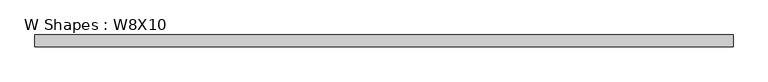
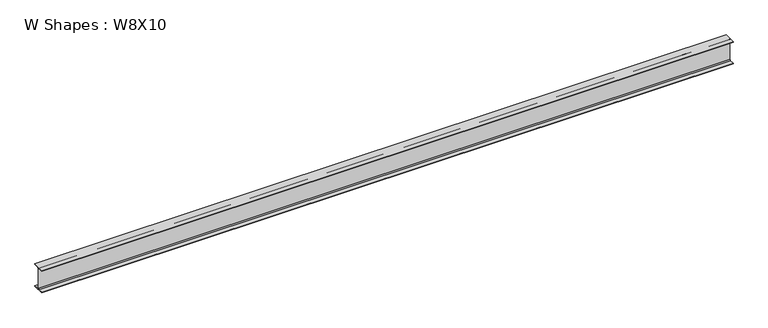
"""IFC4 building model written with IfcOpenShell, lengths in millimetres: beam geometry, W Shapes : W8X10."""

from ifc_helpers import new_model, si_unit, point, frame, frame_2d, origin, place, context, project, spatial, polyline, circle_curve, trimmed, segment, composite_curve, outline, extrude, source, transform, mapped, element, save


def w_shapes_w8x10_5ccd87fd(model_context):
    return source(origin(), model_context, "Body", "SweptSolid", [
        extrude(outline(composite_curve([segment(polyline([(50.038, -94.996), (50.038, -100.203), (-50.038, -100.203), (-50.038, -94.996), (-9.779, -94.996)]), True, "CONTINUOUS"), segment(trimmed(circle_curve(frame_2d((-9.779, -87.376)), 7.62), [point((-9.779, -94.996))], [point((-2.159, -87.376))], True, "CARTESIAN"), True, "CONTINUOUS"), segment(polyline([(-2.159, -87.376), (-2.159, 87.376)]), True, "CONTINUOUS"), segment(trimmed(circle_curve(frame_2d((-9.779, 87.376)), 7.62), [point((-2.159, 87.376))], [point((-9.779, 94.996))], True, "CARTESIAN"), True, "CONTINUOUS"), segment(polyline([(-9.779, 94.996), (-50.038, 94.996), (-50.038, 100.203), (50.038, 100.203), (50.038, 94.996), (9.779, 94.996)]), True, "CONTINUOUS"), segment(trimmed(circle_curve(frame_2d((9.779, 87.376)), 7.62), [point((9.779, 94.996))], [point((2.159, 87.376))], True, "CARTESIAN"), True, "CONTINUOUS"), segment(polyline([(2.159, 87.376), (2.159, -87.376)]), True, "CONTINUOUS"), segment(trimmed(circle_curve(frame_2d((9.779, -87.376)), 7.62), [point((2.159, -87.376))], [point((9.779, -94.996))], True, "CARTESIAN"), True, "CONTINUOUS"), segment(polyline([(9.779, -94.996), (50.038, -94.996)]), True, "CONTINUOUS")], self_intersect=False)), frame((-2950.845, 0.0, 0.0), z_axis=(1.0, 0.0, 0.0), x_axis=(0.0, 1.0, 0.0)), (0.0, 0.0, 1.0), 5901.69),
    ])


if __name__ == "__main__":
    model = new_model("IFC4")
    model_context = context("Model", 3, world=origin())
    ifc_project = project(units=[si_unit("LENGTHUNIT", "METRE", prefix="MILLI")], contexts=[model_context])
    site = spatial("IfcSite", under=ifc_project)
    building = spatial("IfcBuilding", under=site)
    placement = place(None, origin())
    w_shapes_w8x10_shape = w_shapes_w8x10_5ccd87fd(model_context)
    element("IfcBeam", 1, ObjectType="W Shapes : W8X10", at=placement, inside=building, context=model_context, shape_type="MappedRepresentation", body=[
        mapped(w_shapes_w8x10_shape, transform((0.0, 0.0, 0.0), x_axis=(1.0, 0.0, 0.0), y_axis=(0.0, 1.0, 0.0), z_axis=(0.0, 0.0, 1.0))),
    ])
    save(model, "model.ifc")

# Revit data of these elements
# Type "W Shapes : W8X10"
#   Section Name Key = "W8x10"
#   Assembly Code = "B10"
#   Width = 3.940"
#   Web Thickness = 0.170"
#   Web Fillet = 0.300"
#   Warping Constant = 30.90 in⁶
#   Torsional Moment of Inertia = 0.0426 in⁴
#   Section Area = 2.96 in²
#   Plastic Modulus weak axis = 1.66 in³
#   Plastic Modulus strong axis = 8.87 in³
#   Perimeter = 30.70 ft²/ft
#   Nominal Weight = 10.00 lbf/ft
#   Moment of Inertia weak axis = 2.09 in⁴
#   Moment of Inertia strong axis = 30.80 in⁴
#   Height = 7.890"
#   Flange Thickness = 0.205"
#   Elastic Modulus weak axis = 1.06 in³
#   Elastic Modulus strong axis = 7.81 in³
#   Centroid Vertical = 3.945"
#   Centroid Horizontal = 1.970"
#   Bolt Spacing = 0' - 2 1/4"
#   Length [instance default] = 5' - 0"
#   Structural Material [instance default] = Steel ASTM A992
#   Principal Axes Angle = 0
# Element 1 (IfcBeam, "W Shapes : W8X10")
#   Materials on its faces: "Steel ASTM A992"
# Materials
#   "Steel ASTM A992": class "Metal", colour RGB 199 199 199, transparency 0, Description = "Structural steel 50ksi", Cost = 0
